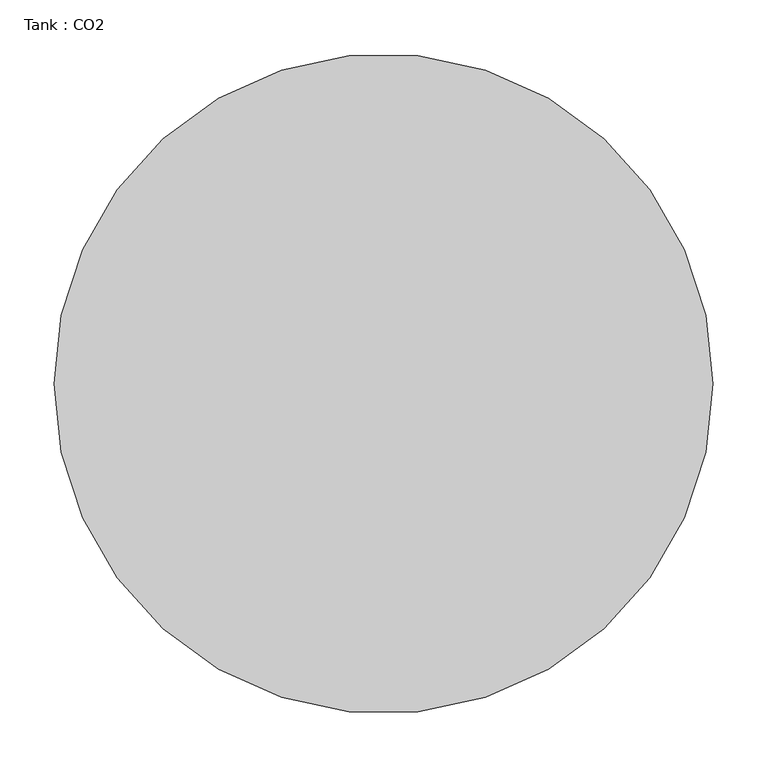
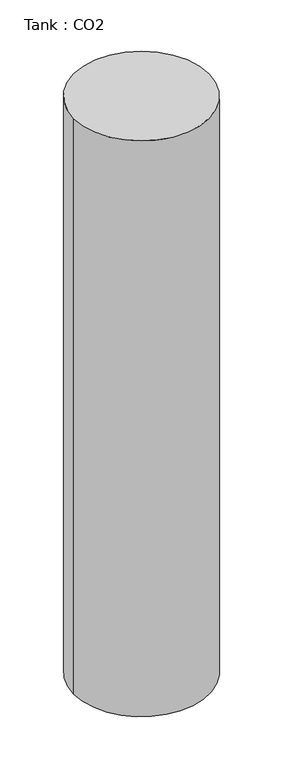
"""IFC4 building model written with IfcOpenShell, lengths in millimetres: proxy geometry, Tank : CO2."""

from ifc_helpers import new_model, si_unit, point, origin, origin_with_axes, origin_2d, place, context, project, spatial, circle_curve, trimmed, segment, composite_curve, outline, extrude, source, transform, mapped, element, save


def tank_co2_4ef1c0a1(model_context):
    return source(origin(), model_context, "Body", "SweptSolid", [
        extrude(outline(composite_curve([segment(trimmed(circle_curve(origin_2d(), 304.8), [point((-304.8, 0.0))], [point((304.8, 0.0))], False, "CARTESIAN"), True, "CONTINUOUS"), segment(trimmed(circle_curve(origin_2d(), 304.8), [point((304.8, 0.0))], [point((-304.8, 0.0))], False, "CARTESIAN"), True, "CONTINUOUS")], self_intersect=False)), origin_with_axes(), (0.0, 0.0, 1.0), 2743.2),
    ])


if __name__ == "__main__":
    model = new_model("IFC4")
    model_context = context("Model", 3, world=origin())
    ifc_project = project(units=[si_unit("LENGTHUNIT", "METRE", prefix="MILLI")], contexts=[model_context])
    site = spatial("IfcSite", under=ifc_project)
    building = spatial("IfcBuilding", under=site)
    placement = place(None, origin())
    tank_co2_shape = tank_co2_4ef1c0a1(model_context)
    element("IfcBuildingElementProxy", 1, Name="Tank : CO2", ObjectType="Tank : CO2", at=placement, inside=building, context=model_context, shape_type="MappedRepresentation", body=[
        mapped(tank_co2_shape, transform((0.0, 0.0, 0.0), x_axis=(1.0, 0.0, 0.0), y_axis=(0.0, 1.0, 0.0), z_axis=(0.0, 0.0, 1.0))),
    ])
    save(model, "model.ifc")

# Revit data of these elements
# Type "Tank : CO2"
#   radius = 1' - 0"
#   Height = 9' - 0"
#   Diameter = 2' - 0"
#   Material = CO2
# Element 1 (IfcBuildingElementProxy, "Tank : CO2")
#   Materials on its faces: "CO2"
# Materials
#   "CO2": class "Generic", colour RGB 181 181 181, transparency 0, Cost = 0
